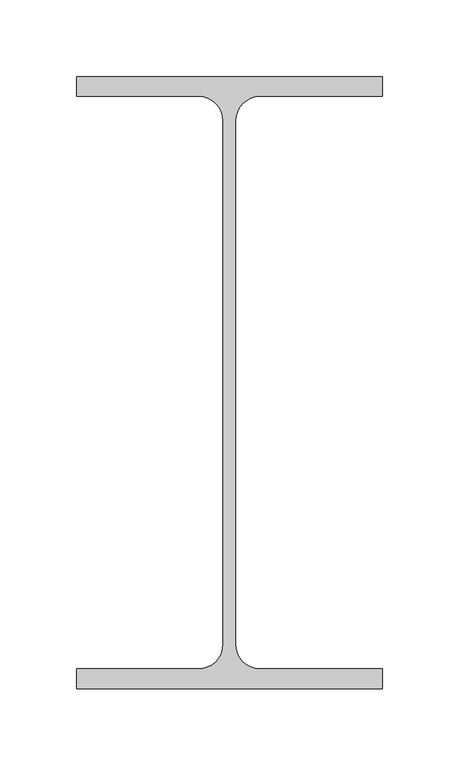
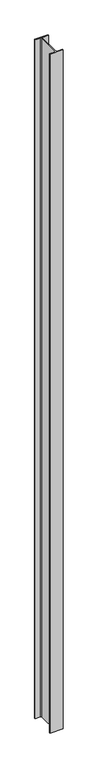
"""IFC4 building model written with IfcOpenShell, lengths in millimetres: column geometry, Steel Column_H_KSD3502 : H_SC_ASC_H-400x200x8x13."""

import ifcopenshell
import ifcopenshell.guid

model = None  # the IFC model being written
_history = None  # IfcOwnerHistory: only IFC2X3 demands one
_inside = {}  # id of a spatial element -> (the spatial element, [elements in it])
_under = {}  # id of a project, library or spatial element -> (it, [spatial elements below it])
_declared = {}  # id of a project -> (the project, [libraries it declares])
_typed = {}  # id of a type object -> (the type object, [elements of that type])
_made_of = {}  # id of a material, layer set ... -> (it, [elements and type objects made of it])


def new_model(schema):
    """Start an empty IFC model of exactly this schema.

    Asked for "IFC4X3", IfcOpenShell would pick the latest addendum, in which some entities
    have other attributes; the version numbers below select the first issue.
    IFC2X3 requires an IfcOwnerHistory on every rooted entity: one is made here for all.
    """
    global model, _history
    if schema == "IFC4X3":
        model = ifcopenshell.file(schema_version=(4, 3, 0, 0))
    else:
        model = ifcopenshell.file(schema=schema)
    _inside.clear()
    _under.clear()
    _declared.clear()
    _typed.clear()
    _made_of.clear()
    _history = None
    if model.schema == "IFC2X3":
        org = make("IfcOrganization", Name="unknown")
        user = make(
            "IfcPersonAndOrganization",
            ThePerson=make("IfcPerson", FamilyName="unknown"),
            TheOrganization=org,
        )
        app = make(
            "IfcApplication",
            ApplicationDeveloper=org,
            Version="unknown",
            ApplicationFullName="unknown",
            ApplicationIdentifier="unknown",
        )
        _history = make(
            "IfcOwnerHistory",
            OwningUser=user,
            OwningApplication=app,
            ChangeAction="ADDED",
            CreationDate=0,
        )
    return model


def make(cls, **values):
    """One entity of the class cls with the attributes given. An attribute that is None is left unset."""
    return model.create_entity(
        cls, **{name: value for name, value in values.items() if value is not None}
    )


def rooted(cls, **values):
    """An entity with a GlobalId (a new one), such as an element, a storey or a relation."""
    return make(cls, GlobalId=ifcopenshell.guid.new(), OwnerHistory=_history, **values)


def si_unit(unit_type, name, prefix=None):
    """IfcSIUnit, for example si_unit("LENGTHUNIT", "METRE", prefix="MILLI")."""
    return make("IfcSIUnit", UnitType=unit_type, Prefix=prefix, Name=name)


def assignment(units):
    """IfcUnitAssignment: the units of a project."""
    return None if units is None else make("IfcUnitAssignment", Units=units)


def point(xyz):
    """IfcCartesianPoint."""
    return None if xyz is None else make("IfcCartesianPoint", Coordinates=xyz)


def direction(xyz):
    """IfcDirection."""
    return None if xyz is None else make("IfcDirection", DirectionRatios=xyz)


def frame(location, z_axis=None, x_axis=None):
    """IfcAxis2Placement3D, a coordinate frame: its origin and axes. An axis left out is left unset."""
    return make(
        "IfcAxis2Placement3D",
        Location=point(location),
        Axis=direction(z_axis),
        RefDirection=direction(x_axis),
    )


def frame_2d(location, x_axis=None):
    """IfcAxis2Placement2D, a coordinate frame in the plane: its origin and x axis."""
    return make(
        "IfcAxis2Placement2D", Location=point(location), RefDirection=direction(x_axis)
    )


def origin():
    """The frame at (0, 0, 0) with its axes left unset."""
    return frame((0.0, 0.0, 0.0))


def place(relative_to, where):
    """IfcLocalPlacement: puts the frame where relative to a parent placement (None: the world)."""
    return make(
        "IfcLocalPlacement", PlacementRelTo=relative_to, RelativePlacement=where
    )


def context(
    kind, dimensions, precision=None, world=None, true_north=None, identifier=None
):
    """IfcGeometricRepresentationContext, for example the 3D "Model" context."""
    return make(
        "IfcGeometricRepresentationContext",
        ContextIdentifier=identifier,
        ContextType=kind,
        CoordinateSpaceDimension=dimensions,
        Precision=precision,
        WorldCoordinateSystem=world,
        TrueNorth=true_north,
    )


def project(units=None, contexts=None):
    """IfcProject with its units and contexts."""
    return rooted(
        "IfcProject",
        Name="project",
        RepresentationContexts=contexts,
        UnitsInContext=assignment(units),
    )


def spatial(cls, under=None, at=None, **own):
    """A site, building, storey or space (cls), placed at a placement, below another one or the project."""
    s = rooted(cls, ObjectPlacement=at, **own)
    if under is not None:
        _under.setdefault(under.id(), (under, []))[1].append(s)
    return s


def polyline(points):
    """IfcPolyline through the points."""
    return make("IfcPolyline", Points=[point(p) for p in points])


def circle_curve(where, radius):
    """IfcCircle in the frame where."""
    return make("IfcCircle", Position=where, Radius=radius)


def trimmed(basis, trim1, trim2, sense, master):
    """IfcTrimmedCurve: the piece of a basis curve between two trims."""
    return make(
        "IfcTrimmedCurve",
        BasisCurve=basis,
        Trim1=trim1,
        Trim2=trim2,
        SenseAgreement=sense,
        MasterRepresentation=master,
    )


def segment(curve, same_sense, transition):
    """IfcCompositeCurveSegment."""
    return make(
        "IfcCompositeCurveSegment",
        Transition=transition,
        SameSense=same_sense,
        ParentCurve=curve,
    )


def composite_curve(segments, self_intersect=None):
    """IfcCompositeCurve: segments joined end to end."""
    return make("IfcCompositeCurve", Segments=segments, SelfIntersect=self_intersect)


def outline(outer, holes=None, kind="AREA"):
    """IfcArbitraryClosedProfileDef: a profile drawn as a closed curve; with holes, ...WithVoids."""
    if holes is None:
        return make("IfcArbitraryClosedProfileDef", ProfileType=kind, OuterCurve=outer)
    return make(
        "IfcArbitraryProfileDefWithVoids",
        ProfileType=kind,
        OuterCurve=outer,
        InnerCurves=holes,
    )


def extrude(swept, where, along, depth):
    """IfcExtrudedAreaSolid: the profile swept, set in the frame where, extruded along a direction by depth."""
    return make(
        "IfcExtrudedAreaSolid",
        SweptArea=swept,
        Position=where,
        ExtrudedDirection=direction(along),
        Depth=depth,
    )


def shape(context_of_items, identifier, shape_type, items):
    """IfcShapeRepresentation: the items that make up one representation, for example the "Body"."""
    return make(
        "IfcShapeRepresentation",
        ContextOfItems=context_of_items,
        RepresentationIdentifier=identifier,
        RepresentationType=shape_type,
        Items=items,
    )


def source(mapping_origin, context_of_items, identifier, shape_type, items):
    """IfcRepresentationMap: a shape defined once, which mapped items show again and again."""
    return make(
        "IfcRepresentationMap",
        MappingOrigin=mapping_origin,
        MappedRepresentation=shape(context_of_items, identifier, shape_type, items),
    )


def transform(
    local_origin,
    x_axis=None,
    y_axis=None,
    z_axis=None,
    scale=None,
    scale2=None,
    scale3=None,
    uniform=True,
):
    """IfcCartesianTransformationOperator3D, or its non-uniform kind. x_axis, y_axis, z_axis: its Axis1, 2, 3."""
    if uniform:
        return make(
            "IfcCartesianTransformationOperator3D",
            Axis1=direction(x_axis),
            Axis2=direction(y_axis),
            LocalOrigin=point(local_origin),
            Scale=scale,
            Axis3=direction(z_axis),
        )
    return make(
        "IfcCartesianTransformationOperator3DnonUniform",
        Axis1=direction(x_axis),
        Axis2=direction(y_axis),
        LocalOrigin=point(local_origin),
        Scale=scale,
        Axis3=direction(z_axis),
        Scale2=scale2,
        Scale3=scale3,
    )


def mapped(mapping_source, mapping_target):
    """IfcMappedItem: shows the shape of a source again, moved by a transform."""
    return make(
        "IfcMappedItem", MappingSource=mapping_source, MappingTarget=mapping_target
    )


def made_of(thing, what):
    """Note that an element or type object is made of a material, layer set ...; save() writes the relation."""
    if what is not None:
        _made_of.setdefault(what.id(), (what, []))[1].append(thing)
    return thing


def element(
    cls,
    number,
    at=None,
    inside=None,
    cuts=None,
    type_object=None,
    material=None,
    context=None,
    identifier="Body",
    shape_type=None,
    held_by="IfcProductDefinitionShape",
    body=None,
    shapes=None,
    **own,
):
    """One element of the class cls, such as IfcWall. Its Tag is "e" and its number.

    at: its placement. inside: the storey or other place that contains it. cuts: it is an
    opening in that element (IfcRelVoidsElement). A single representation is given by context,
    identifier, shape_type and body (its items); several are given by shapes. held_by: the class
    of the entity that holds the representations. save() writes the other relations.
    """
    e = rooted(cls, Tag="e%d" % number, ObjectPlacement=at, **own)
    if body is not None:
        shapes = [shape(context, identifier, shape_type, body)]
    if shapes is not None:
        e.Representation = make(held_by, Representations=shapes)
    if inside is not None:
        _inside.setdefault(inside.id(), (inside, []))[1].append(e)
    if cuts is not None:
        rooted(
            "IfcRelVoidsElement", RelatingBuildingElement=cuts, RelatedOpeningElement=e
        )
    if type_object is not None:
        _typed.setdefault(type_object.id(), (type_object, []))[1].append(e)
    return made_of(e, material)


def aggregate(whole, parts):
    """IfcRelAggregates: a whole, such as a stair, and the parts it consists of."""
    return rooted("IfcRelAggregates", RelatingObject=whole, RelatedObjects=parts)


def save(model, path):
    """Write the relations noted so far, then the file.

    IfcRelAggregates (storeys below a building ...), IfcRelContainedInSpatialStructure (elements
    in a storey), IfcRelDefinesByType, IfcRelAssociatesMaterial and IfcRelDeclares: one each for
    every whole, place, type object, material and project.
    """
    for whole, parts in _under.values():
        aggregate(whole, parts)
    for where, things in _inside.values():
        rooted(
            "IfcRelContainedInSpatialStructure",
            RelatedElements=things,
            RelatingStructure=where,
        )
    for kind, things in _typed.values():
        rooted("IfcRelDefinesByType", RelatedObjects=things, RelatingType=kind)
    for what, things in _made_of.values():
        rooted("IfcRelAssociatesMaterial", RelatedObjects=things, RelatingMaterial=what)
    for by, libraries in _declared.values():
        rooted("IfcRelDeclares", RelatingContext=by, RelatedDefinitions=libraries)
    model.write(path)


def column_8add4d16(model_context):
    return source(origin(), model_context, "Body", "SweptSolid", [
        extrude(outline(composite_curve([segment(polyline([(100.0, 200.0), (100.0, 187.0), (20.0, 187.0)]), True, "CONTINUOUS"), segment(trimmed(circle_curve(frame_2d((20.0, 171.0)), 16.0), [point((20.0, 187.0))], [point((4.0, 171.0))], True, "CARTESIAN"), True, "CONTINUOUS"), segment(polyline([(4.0, 171.0), (4.0, -171.0)]), True, "CONTINUOUS"), segment(trimmed(circle_curve(frame_2d((20.0, -171.0)), 16.0), [point((4.0, -171.0))], [point((20.0, -187.0))], True, "CARTESIAN"), True, "CONTINUOUS"), segment(polyline([(20.0, -187.0), (100.0, -187.0), (100.0, -200.0), (-100.0, -200.0), (-100.0, -187.0), (-20.0, -187.0)]), True, "CONTINUOUS"), segment(trimmed(circle_curve(frame_2d((-20.0, -171.0)), 16.0), [point((-20.0, -187.0))], [point((-4.0, -171.0))], True, "CARTESIAN"), True, "CONTINUOUS"), segment(polyline([(-4.0, -171.0), (-4.0, 171.0)]), True, "CONTINUOUS"), segment(trimmed(circle_curve(frame_2d((-20.0, 171.0)), 16.0), [point((-4.0, 171.0))], [point((-20.0, 187.0))], True, "CARTESIAN"), True, "CONTINUOUS"), segment(polyline([(-20.0, 187.0), (-100.0, 187.0), (-100.0, 200.0), (100.0, 200.0)]), True, "CONTINUOUS")], self_intersect=False)), frame((0.0, 0.0, 7249.9720055), z_axis=(0.0, 0.0, 1.0), x_axis=(1.0, 0.0, 0.0)), (0.0, 0.0, 1.0), 10950.0),
    ])


if __name__ == "__main__":
    model = new_model("IFC4")
    model_context = context("Model", 3, world=origin())
    ifc_project = project(units=[si_unit("LENGTHUNIT", "METRE", prefix="MILLI")], contexts=[model_context])
    site = spatial("IfcSite", under=ifc_project)
    building = spatial("IfcBuilding", under=site)
    placement = place(None, origin())
    column_shape = column_8add4d16(model_context)
    element("IfcColumn", 1, ObjectType="Steel Column_H_KSD3502 : H_SC_ASC_H-400x200x8x13", at=placement, inside=building, context=model_context, shape_type="MappedRepresentation", body=[
        mapped(column_shape, transform((0.0, 0.0, 0.0), x_axis=(1.0, 0.0, 0.0), y_axis=(0.0, 1.0, 0.0), z_axis=(0.0, 0.0, 1.0))),
    ])
    save(model, "model.ifc")

# Revit data of these elements
# Type "Steel Column_H_KSD3502 : H_SC_ASC_H-400x200x8x13"
#   Width = 20.0 cm
#   Web Thickness = 0.8 cm
#   Web Fillet = 1.6 cm
#   Warping Constant = 648999.0 cm⁶
#   Torsional Moment of Inertia = 35.8981 cm⁴
#   Section Area = 84.12 cm²
#   Plastic Modulus weak axis = 268.0 cm³
#   Plastic Modulus strong axis = 1330.0 cm³
#   Perimeter = 1.27 m²/m
#   Nominal Weight = 66.00 kgf/m
#   Moment of Inertia weak axis = 1740.00 cm⁴
#   Moment of Inertia strong axis = 23700.00 cm⁴
#   Height = 40.0 cm
#   Flange Thickness = 1.3 cm
#   Elastic Modulus weak axis = 174.0 cm³
#   Elastic Modulus strong axis = 1190.0 cm³
#   Centroid Vertical = 20.0 cm
#   Centroid Horizontal = 10.0 cm
#   Bolt Spacing = 13.97 cm
#   Structural Material [instance default] = Steel, 45-345
#   Section Name Key = ""
#   Assembly Code = ""
# Element 1 (IfcColumn, "Steel Column_H_KSD3502 : H_SC_ASC_H-400x200x8x13")
#   Structural Material = none
# Materials
#   "Steel, 45-345": class "Metal", colour RGB 189 187 185, transparency 0, Description = "Steel 345 MPa", Cost = 0
